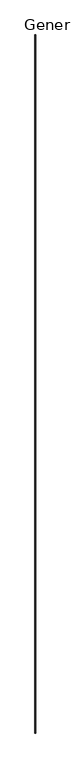
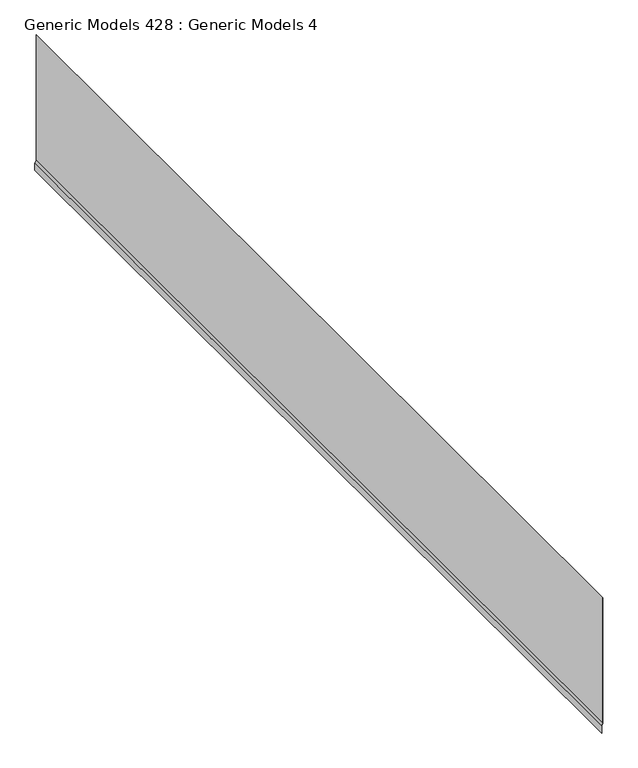
"""IFC4 building model written with IfcOpenShell, lengths in millimetres: proxy geometry, Generic Models 428 : Generic Models 4."""

from ifc_helpers import new_model, si_unit, origin, place, context, project, spatial, faceted_brep, source, transform, mapped, element, save


def generic_models_428_generic_models_4_d5f69094(model_context):
    return source(origin(), model_context, "Body", "Brep", [
        faceted_brep([(-6631.7360956, -6864.9230338, 129263.2444381), (-6631.7360956, -6864.9230338, 130126.2313356), (-6632.5298456, -6864.9230338, 130126.2313356), (-6632.5298456, -6864.9230338, 129263.3843976), (-6638.0717238, -6864.9230338, 129248.1582124), (-6639.9535719, -6864.9230338, 129242.9878771), (-6639.9535719, -6864.9230338, 129196.8879493), (-6639.1598219, -6864.9230338, 129196.8879493), (-6639.1598219, -6864.9230338, 129242.8479176), (-6638.0717238, -6864.9230338, 129245.8374426), (-6631.7360956, -464.1230338, 129263.2444381), (-6638.0717238, -464.1230338, 129245.8374426), (-6639.1598219, -464.1230338, 129242.8479176), (-6639.1598219, -464.1230338, 129196.8879493), (-6639.9535719, -464.1230338, 129196.8879493), (-6639.9535719, -464.1230338, 129242.9878771), (-6638.0717238, -464.1230338, 129248.1582124), (-6632.5298456, -464.1230338, 129263.3843976), (-6632.5298456, -464.1230338, 130126.2313356), (-6631.7360956, -464.1230338, 130126.2313356)], [[[0, 1, 2, 3, 4, 5, 6, 7, 8, 9]], [[10, 11, 12, 13, 14, 15, 16, 17, 18, 19]], [[1, 0, 10, 19]], [[0, 9, 8, 12, 11, 10]], [[8, 7, 13, 12]], [[7, 6, 14, 13]], [[6, 5, 15, 14]], [[5, 4, 3, 17, 16, 15]], [[3, 2, 18, 17]], [[2, 1, 19, 18]]]),
    ])


if __name__ == "__main__":
    model = new_model("IFC4")
    model_context = context("Model", 3, world=origin())
    ifc_project = project(units=[si_unit("LENGTHUNIT", "METRE", prefix="MILLI")], contexts=[model_context])
    site = spatial("IfcSite", under=ifc_project)
    building = spatial("IfcBuilding", under=site)
    placement = place(None, origin())
    generic_models_428_generic_models_4_shape = generic_models_428_generic_models_4_d5f69094(model_context)
    element("IfcBuildingElementProxy", 1, Name="Generic Models 428 : Generic Models 4", ObjectType="Generic Models 428 : Generic Models 4", at=placement, inside=building, context=model_context, shape_type="MappedRepresentation", body=[
        mapped(generic_models_428_generic_models_4_shape, transform((0.0, 0.0, 0.0), x_axis=(1.0, 0.0, 0.0), y_axis=(0.0, 1.0, 0.0), z_axis=(0.0, 0.0, 1.0))),
    ])
    save(model, "model.ifc")

# Revit data of these elements
# Element 1 (IfcBuildingElementProxy, "Generic Models 428 : Generic Models 4")
#   Materials on its faces: "_(2) LAYERS NO. 30 ASTM D226 ASPHALT SATURATED ORGANIC FELT"
# Materials
#   "_(2) LAYERS NO. 30 ASTM D226 ASPHALT SATURATED ORGANIC FELT": class "Generic", colour RGB 67 154 161, transparency 0, Cost = 0
